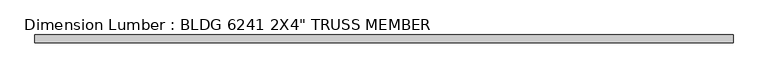
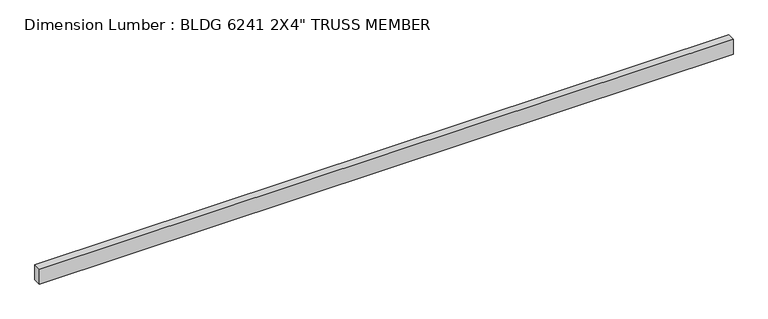
"""IFC4 building model written with IfcOpenShell, lengths in millimetres: beam geometry."""

from ifc_helpers import new_model, si_unit, frame, origin, place, context, project, spatial, polyline, outline, extrude, source, transform, mapped, element, save


def beam_f884bc05(model_context):
    return source(origin(), model_context, "Body", "SweptSolid", [
        extrude(outline(polyline([(2235.2, 25.4), (2235.2, -25.4), (-2235.1999994, -25.4), (-2235.1999994, 25.4), (2235.2, 25.4)])), frame((0.0, 0.0, -50.8), z_axis=(0.0, 0.0, 1.0), x_axis=(1.0, 0.0, 0.0)), (0.0, 0.0, 1.0), 101.6),
    ])


if __name__ == "__main__":
    model = new_model("IFC4")
    model_context = context("Model", 3, world=origin())
    ifc_project = project(units=[si_unit("LENGTHUNIT", "METRE", prefix="MILLI")], contexts=[model_context])
    site = spatial("IfcSite", under=ifc_project)
    building = spatial("IfcBuilding", under=site)
    placement = place(None, origin())
    beam_shape = beam_f884bc05(model_context)
    element("IfcBeam", 1, ObjectType="Dimension Lumber : BLDG 6241 2X4\" TRUSS MEMBER", at=placement, inside=building, context=model_context, shape_type="MappedRepresentation", body=[
        mapped(beam_shape, transform((0.0, 0.0, 0.0), x_axis=(1.0, 0.0, 0.0), y_axis=(0.0, 1.0, 0.0), z_axis=(0.0, 0.0, 1.0))),
    ])
    save(model, "model.ifc")

# Revit data of these elements
# Type "Dimension Lumber : BLDG 6241 2X4\" TRUSS MEMBER"
#   Assembly Code = "B10"
#   A = 0.273472 SF
#   Length [instance default] = 5' - 0"
#   b = 0' - 2"
#   d = 0' - 4"
#   Structural Material [instance default] = Softwood, Lumber
# Element 1 (IfcBeam, "Dimension Lumber : BLDG 6241 2X4\" TRUSS MEMBER")
#   Materials on its faces: "Softwood, Lumber"
# Materials
#   "Softwood, Lumber": class "Wood", colour RGB 223 192 134, transparency 0, Description = "Pinus Echinata", Cost = 0
